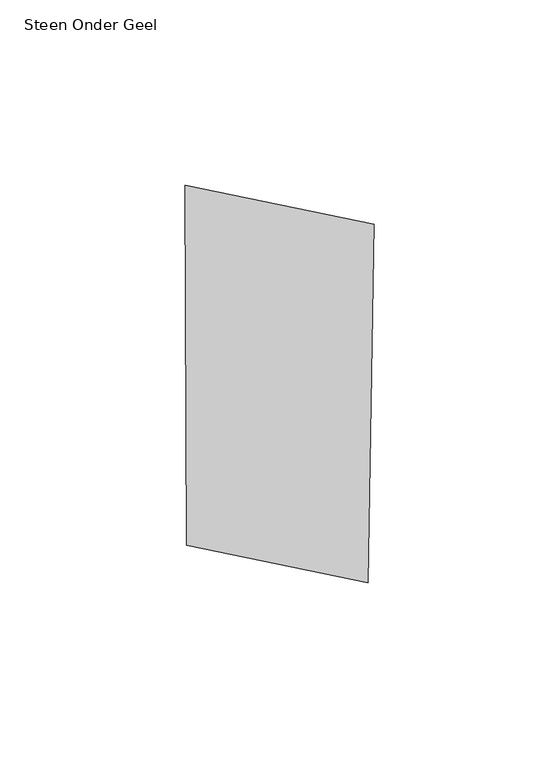
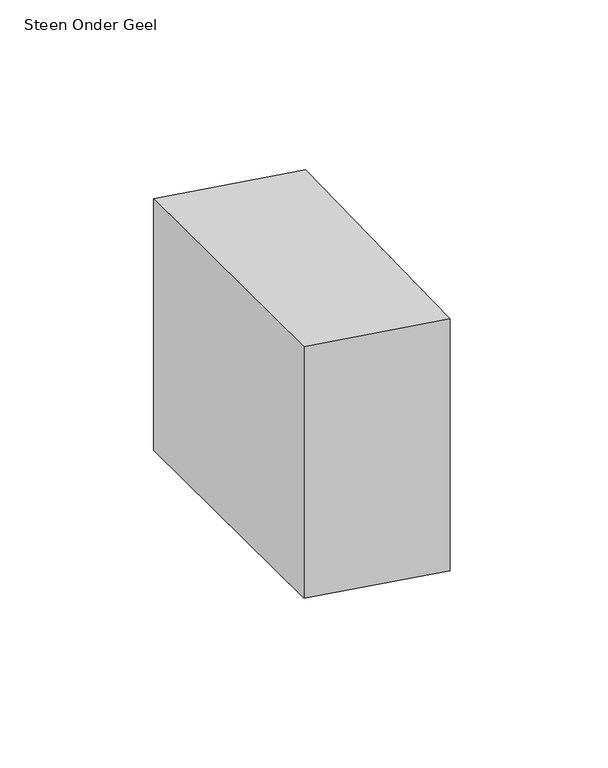
"""IFC4 building model written with IfcOpenShell, lengths in millimetres: proxy geometry, 00_GMA_steen_versie_4 : Steen Onder Geel."""

from ifc_helpers import new_model, si_unit, origin, origin_with_axes, place, context, project, spatial, polyline, outline, extrude, source, transform, mapped, element, save


def steen_onder_geel_71faef55(model_context):
    return source(origin(), model_context, "Body", "SweptSolid", [
        extrude(outline(polyline([(101.4319988, 115.486472), (99.7966444, 18.7303184), (50.829255, 28.8394612), (50.3944284, 126.0409435), (101.4319988, 115.486472)])), origin_with_axes(), (0.0, 0.0, 1.0), 100.0),
    ])


if __name__ == "__main__":
    model = new_model("IFC4")
    model_context = context("Model", 3, world=origin())
    ifc_project = project(units=[si_unit("LENGTHUNIT", "METRE", prefix="MILLI")], contexts=[model_context])
    site = spatial("IfcSite", under=ifc_project)
    building = spatial("IfcBuilding", under=site)
    placement = place(None, origin())
    steen_onder_geel_shape = steen_onder_geel_71faef55(model_context)
    element("IfcBuildingElementProxy", 1, Name="00_GMA_steen_versie_4 : Steen Onder Geel", ObjectType="00_GMA_steen_versie_4 : Steen Onder Geel", at=placement, inside=building, context=model_context, shape_type="MappedRepresentation", body=[
        mapped(steen_onder_geel_shape, transform((0.0, 0.0, 0.0), x_axis=(1.0, 0.0, 0.0), y_axis=(0.0, 1.0, 0.0), z_axis=(0.0, 0.0, 1.0))),
    ])
    save(model, "model.ifc")

# Revit data of these elements
# Type "00_GMA_steen_versie_4 : Steen Onder Geel"
#   StootVoegHalfBoven [instance default] = 5 mm
#   StootVoegHalf [instance default] = 5 mm
#   StootVoegBreedteOnder = 10 mm
#   StootVoegBreedteBoven = 10 mm
#   Steendikte = 100 mm
#   LintVoegOnderHalf = 0 mm
#   LintVoegOnder = 0 mm
#   LintVoegBovenHalf = 5 mm
#   LintVoegBoven = 10 mm
#   materiaal = 21_steen_geel
#   MateriaalVoeg = none
#   Default Elevation = 0
# Element 1 (IfcBuildingElementProxy, "00_GMA_steen_versie_4 : Steen Onder Geel")
#   Materials on its faces: "21_steen_geel"
# Materials
#   "21_steen_geel": class "Unassigned", colour RGB 202 202 0, transparency 0, Cost = 0
